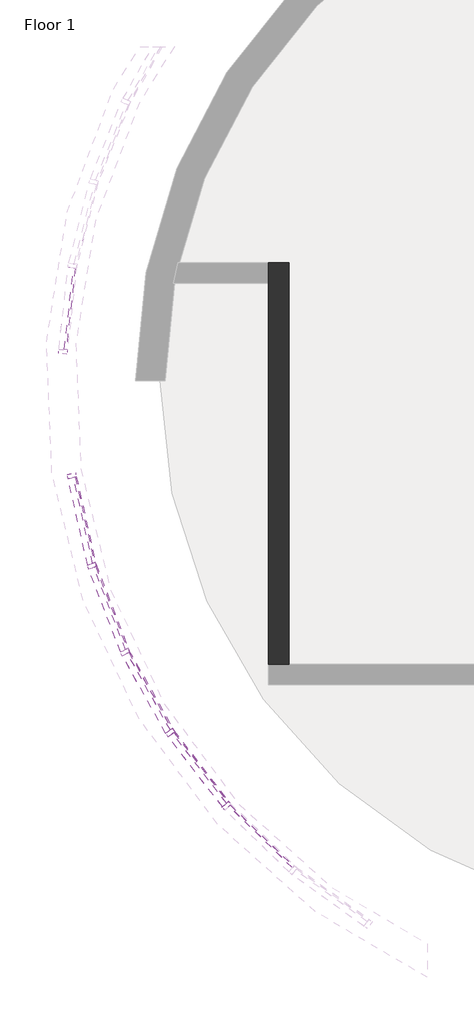
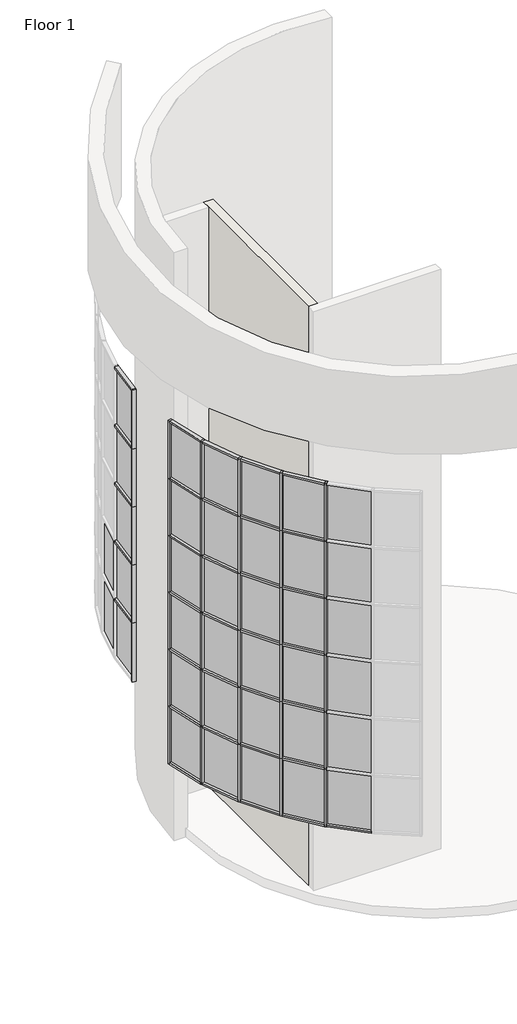
# One storey, part 1 of 11: 69 members, 37 plates, 1 wall.
"""IFC4 building model written with IfcOpenShell, lengths in millimetres."""

import ifcopenshell
import ifcopenshell.guid

model = None  # the IFC model being written
_history = None  # IfcOwnerHistory: only IFC2X3 demands one
_inside = {}  # id of a spatial element -> (the spatial element, [elements in it])
_under = {}  # id of a project, library or spatial element -> (it, [spatial elements below it])
_declared = {}  # id of a project -> (the project, [libraries it declares])
_typed = {}  # id of a type object -> (the type object, [elements of that type])
_made_of = {}  # id of a material, layer set ... -> (it, [elements and type objects made of it])


def new_model(schema):
    """Start an empty IFC model of exactly this schema.

    Asked for "IFC4X3", IfcOpenShell would pick the latest addendum, in which some entities
    have other attributes; the version numbers below select the first issue.
    IFC2X3 requires an IfcOwnerHistory on every rooted entity: one is made here for all.
    """
    global model, _history
    if schema == "IFC4X3":
        model = ifcopenshell.file(schema_version=(4, 3, 0, 0))
    else:
        model = ifcopenshell.file(schema=schema)
    _inside.clear()
    _under.clear()
    _declared.clear()
    _typed.clear()
    _made_of.clear()
    _history = None
    if model.schema == "IFC2X3":
        org = make("IfcOrganization", Name="unknown")
        user = make(
            "IfcPersonAndOrganization",
            ThePerson=make("IfcPerson", FamilyName="unknown"),
            TheOrganization=org,
        )
        app = make(
            "IfcApplication",
            ApplicationDeveloper=org,
            Version="unknown",
            ApplicationFullName="unknown",
            ApplicationIdentifier="unknown",
        )
        _history = make(
            "IfcOwnerHistory",
            OwningUser=user,
            OwningApplication=app,
            ChangeAction="ADDED",
            CreationDate=0,
        )
    return model


def make(cls, **values):
    """One entity of the class cls with the attributes given. An attribute that is None is left unset."""
    return model.create_entity(
        cls, **{name: value for name, value in values.items() if value is not None}
    )


def rooted(cls, **values):
    """An entity with a GlobalId (a new one), such as an element, a storey or a relation."""
    return make(cls, GlobalId=ifcopenshell.guid.new(), OwnerHistory=_history, **values)


def si_unit(unit_type, name, prefix=None):
    """IfcSIUnit, for example si_unit("LENGTHUNIT", "METRE", prefix="MILLI")."""
    return make("IfcSIUnit", UnitType=unit_type, Prefix=prefix, Name=name)


def assignment(units):
    """IfcUnitAssignment: the units of a project."""
    return None if units is None else make("IfcUnitAssignment", Units=units)


def point(xyz):
    """IfcCartesianPoint."""
    return None if xyz is None else make("IfcCartesianPoint", Coordinates=xyz)


def direction(xyz):
    """IfcDirection."""
    return None if xyz is None else make("IfcDirection", DirectionRatios=xyz)


def frame(location, z_axis=None, x_axis=None):
    """IfcAxis2Placement3D, a coordinate frame: its origin and axes. An axis left out is left unset."""
    return make(
        "IfcAxis2Placement3D",
        Location=point(location),
        Axis=direction(z_axis),
        RefDirection=direction(x_axis),
    )


def origin():
    """The frame at (0, 0, 0) with its axes left unset."""
    return frame((0.0, 0.0, 0.0))


def origin_with_axes():
    """The frame at (0, 0, 0) with the z axis (0, 0, 1) and the x axis (1, 0, 0) written out."""
    return frame((0.0, 0.0, 0.0), z_axis=(0.0, 0.0, 1.0), x_axis=(1.0, 0.0, 0.0))


def place(relative_to, where):
    """IfcLocalPlacement: puts the frame where relative to a parent placement (None: the world)."""
    return make(
        "IfcLocalPlacement", PlacementRelTo=relative_to, RelativePlacement=where
    )


def context(
    kind, dimensions, precision=None, world=None, true_north=None, identifier=None
):
    """IfcGeometricRepresentationContext, for example the 3D "Model" context."""
    return make(
        "IfcGeometricRepresentationContext",
        ContextIdentifier=identifier,
        ContextType=kind,
        CoordinateSpaceDimension=dimensions,
        Precision=precision,
        WorldCoordinateSystem=world,
        TrueNorth=true_north,
    )


def project(units=None, contexts=None):
    """IfcProject with its units and contexts."""
    return rooted(
        "IfcProject",
        Name="project",
        RepresentationContexts=contexts,
        UnitsInContext=assignment(units),
    )


def spatial(cls, under=None, at=None, **own):
    """A site, building, storey or space (cls), placed at a placement, below another one or the project."""
    s = rooted(cls, ObjectPlacement=at, **own)
    if under is not None:
        _under.setdefault(under.id(), (under, []))[1].append(s)
    return s


def polyline(points):
    """IfcPolyline through the points."""
    return make("IfcPolyline", Points=[point(p) for p in points])


def outline(outer, holes=None, kind="AREA"):
    """IfcArbitraryClosedProfileDef: a profile drawn as a closed curve; with holes, ...WithVoids."""
    if holes is None:
        return make("IfcArbitraryClosedProfileDef", ProfileType=kind, OuterCurve=outer)
    return make(
        "IfcArbitraryProfileDefWithVoids",
        ProfileType=kind,
        OuterCurve=outer,
        InnerCurves=holes,
    )


def extrude(swept, where, along, depth):
    """IfcExtrudedAreaSolid: the profile swept, set in the frame where, extruded along a direction by depth."""
    return make(
        "IfcExtrudedAreaSolid",
        SweptArea=swept,
        Position=where,
        ExtrudedDirection=direction(along),
        Depth=depth,
    )


def faces_of(points, faces, orient=None, outer=None):
    """IfcFace entities. A face is a list of loops; a loop is a list of indices into points, from 0.

    orient and outer hold one flag for each loop. By default every Orientation is true, the
    first loop of a face is its IfcFaceOuterBound and the others are IfcFaceBound.
    """
    made = []
    for i, loops in enumerate(faces):
        bounds = []
        for j, loop in enumerate(loops):
            is_outer = j == 0 if outer is None else outer[i][j]
            bounds.append(
                make(
                    "IfcFaceOuterBound" if is_outer else "IfcFaceBound",
                    Bound=make("IfcPolyLoop", Polygon=[points[k] for k in loop]),
                    Orientation=True if orient is None else orient[i][j],
                )
            )
        made.append(make("IfcFace", Bounds=bounds))
    return made


def faceted_brep(points, faces, orient=None, outer=None, voids=None):
    """IfcFacetedBrep: a solid bounded by flat faces; with voids (closed shells), ...WithVoids."""
    shared = [point(p) for p in points]
    hull = make("IfcClosedShell", CfsFaces=faces_of(shared, faces, orient, outer))
    if voids is None:
        return make("IfcFacetedBrep", Outer=hull)
    return make(
        "IfcFacetedBrepWithVoids",
        Outer=hull,
        Voids=[
            make(cls, CfsFaces=faces_of(shared, fs, o, b)) for cls, fs, o, b in voids
        ],
    )


def shape(context_of_items, identifier, shape_type, items):
    """IfcShapeRepresentation: the items that make up one representation, for example the "Body"."""
    return make(
        "IfcShapeRepresentation",
        ContextOfItems=context_of_items,
        RepresentationIdentifier=identifier,
        RepresentationType=shape_type,
        Items=items,
    )


def source(mapping_origin, context_of_items, identifier, shape_type, items):
    """IfcRepresentationMap: a shape defined once, which mapped items show again and again."""
    return make(
        "IfcRepresentationMap",
        MappingOrigin=mapping_origin,
        MappedRepresentation=shape(context_of_items, identifier, shape_type, items),
    )


def transform(
    local_origin,
    x_axis=None,
    y_axis=None,
    z_axis=None,
    scale=None,
    scale2=None,
    scale3=None,
    uniform=True,
):
    """IfcCartesianTransformationOperator3D, or its non-uniform kind. x_axis, y_axis, z_axis: its Axis1, 2, 3."""
    if uniform:
        return make(
            "IfcCartesianTransformationOperator3D",
            Axis1=direction(x_axis),
            Axis2=direction(y_axis),
            LocalOrigin=point(local_origin),
            Scale=scale,
            Axis3=direction(z_axis),
        )
    return make(
        "IfcCartesianTransformationOperator3DnonUniform",
        Axis1=direction(x_axis),
        Axis2=direction(y_axis),
        LocalOrigin=point(local_origin),
        Scale=scale,
        Axis3=direction(z_axis),
        Scale2=scale2,
        Scale3=scale3,
    )


def mapped(mapping_source, mapping_target):
    """IfcMappedItem: shows the shape of a source again, moved by a transform."""
    return make(
        "IfcMappedItem", MappingSource=mapping_source, MappingTarget=mapping_target
    )


def made_of(thing, what):
    """Note that an element or type object is made of a material, layer set ...; save() writes the relation."""
    if what is not None:
        _made_of.setdefault(what.id(), (what, []))[1].append(thing)
    return thing


def element(
    cls,
    number,
    at=None,
    inside=None,
    cuts=None,
    type_object=None,
    material=None,
    context=None,
    identifier="Body",
    shape_type=None,
    held_by="IfcProductDefinitionShape",
    body=None,
    shapes=None,
    **own,
):
    """One element of the class cls, such as IfcWall. Its Tag is "e" and its number.

    at: its placement. inside: the storey or other place that contains it. cuts: it is an
    opening in that element (IfcRelVoidsElement). A single representation is given by context,
    identifier, shape_type and body (its items); several are given by shapes. held_by: the class
    of the entity that holds the representations. save() writes the other relations.
    """
    e = rooted(cls, Tag="e%d" % number, ObjectPlacement=at, **own)
    if body is not None:
        shapes = [shape(context, identifier, shape_type, body)]
    if shapes is not None:
        e.Representation = make(held_by, Representations=shapes)
    if inside is not None:
        _inside.setdefault(inside.id(), (inside, []))[1].append(e)
    if cuts is not None:
        rooted(
            "IfcRelVoidsElement", RelatingBuildingElement=cuts, RelatedOpeningElement=e
        )
    if type_object is not None:
        _typed.setdefault(type_object.id(), (type_object, []))[1].append(e)
    return made_of(e, material)


def aggregate(whole, parts):
    """IfcRelAggregates: a whole, such as a stair, and the parts it consists of."""
    return rooted("IfcRelAggregates", RelatingObject=whole, RelatedObjects=parts)


def save(model, path):
    """Write the relations noted so far, then the file.

    IfcRelAggregates (storeys below a building ...), IfcRelContainedInSpatialStructure (elements
    in a storey), IfcRelDefinesByType, IfcRelAssociatesMaterial and IfcRelDeclares: one each for
    every whole, place, type object, material and project.
    """
    for whole, parts in _under.values():
        aggregate(whole, parts)
    for where, things in _inside.values():
        rooted(
            "IfcRelContainedInSpatialStructure",
            RelatedElements=things,
            RelatingStructure=where,
        )
    for kind, things in _typed.values():
        rooted("IfcRelDefinesByType", RelatedObjects=things, RelatingType=kind)
    for what, things in _made_of.values():
        rooted("IfcRelAssociatesMaterial", RelatedObjects=things, RelatingMaterial=what)
    for by, libraries in _declared.values():
        rooted("IfcRelDeclares", RelatingContext=by, RelatedDefinitions=libraries)
    model.write(path)


def member_2ae322fc(model_context):
    return source(origin(), model_context, "Body", "SweptSolid", [
        extrude(outline(polyline([(-63.5, 0.0), (63.5, 0.0), (63.5, -1253.5867756), (-61.1522336, -1244.9455147), (-63.5, -1278.8126009), (-63.5, 0.0)])), frame((-63.5, 0.0, 0.0), z_axis=(1.0, 0.0, 0.0), x_axis=(0.0, 1.0, 0.0)), (0.0, 0.0, 1.0), 63.5),
    ])


def member_21287d99(model_context):
    return source(origin(), model_context, "Body", "Brep", [
        faceted_brep([(31.75, 63.5, 0.0), (-31.75, 63.5, 0.0), (-31.75, -63.5, 0.0), (31.75, -63.5, 0.0), (31.75, 63.5, -1253.5867756), (0.0, 63.5, -1253.5867756), (-31.75, 63.5, -1253.5867756), (-31.75, -61.1522336, -1244.9455147), (-31.75, -63.5, -1278.8126009), (0.0, -63.5, -1278.8126009), (31.75, -63.5, -1278.8126009), (31.75, -61.1522336, -1244.9455147), (0.0, -61.1522336, -1244.9455147)], [[[0, 1, 2, 3]], [[1, 0, 4, 5, 6]], [[2, 1, 6, 7, 8]], [[3, 2, 8, 9, 10]], [[0, 3, 10, 11, 4]], [[4, 11, 12, 5]], [[11, 10, 9, 12]], [[9, 8, 7, 12]], [[7, 6, 5, 12]]]),
    ])


def member_2f5ef470(model_context):
    return source(origin(), model_context, "Body", "SweptSolid", [
        extrude(outline(polyline([(-63.5, 0.0), (63.5, 0.0), (63.5, -1344.0500431), (-60.9736199, -1334.8041085), (-63.5, -1368.815562), (-63.5, 0.0)])), frame((-63.5, 0.0, 0.0), z_axis=(1.0, 0.0, 0.0), x_axis=(0.0, 1.0, 0.0)), (0.0, 0.0, 1.0), 63.5),
    ])


def member_58fb4e6d(model_context):
    return source(origin(), model_context, "Body", "SweptSolid", [
        extrude(outline(polyline([(-63.5, 29.3948455), (-60.9736199, -4.616608), (63.5, 4.6293267), (63.5, -1339.4207165), (-63.5, -1339.4207165), (-63.5, 29.3948455)])), frame((-63.5, 0.0, 0.0), z_axis=(1.0, 0.0, 0.0), x_axis=(0.0, 1.0, 0.0)), (0.0, 0.0, 1.0), 63.5),
    ])


def member_233ab79f(model_context):
    return source(origin(), model_context, "Body", "SweptSolid", [
        extrude(outline(polyline([(-63.5, 29.4471051), (-61.0333155, -4.5163328), (63.5, 4.5282284), (63.5, -1343.9489353), (-61.0333155, -1334.904374), (-63.5, -1368.8678119), (-63.5, 29.4471051)])), frame((-63.5, 0.0, 0.0), z_axis=(1.0, 0.0, 0.0), x_axis=(0.0, 1.0, 0.0)), (0.0, 0.0, 1.0), 63.5),
    ])


def member_23db0025(model_context):
    return source(origin(), model_context, "Body", "Brep", [
        faceted_brep([(31.75, 63.5, -1339.4207165), (31.75, -63.5, -1339.4207165), (-31.75, -63.5, -1339.4207165), (-31.75, 63.5, -1339.4207165), (-31.75, 63.5, 4.6293267), (0.0, 63.5, 4.6293267), (31.75, 63.5, 4.6293267), (-31.75, -63.5, 29.3948455), (-31.75, -60.9736199, -4.616608), (31.75, -63.5, 29.3948455), (0.0, -63.5, 29.3948455), (31.75, -60.9736199, -4.616608), (0.0, -60.9736199, -4.616608)], [[[0, 1, 2, 3]], [[4, 5, 6, 0, 3]], [[7, 8, 4, 3, 2]], [[9, 10, 7, 2, 1]], [[6, 11, 9, 1, 0]], [[6, 5, 12, 11]], [[5, 4, 8, 12]], [[8, 7, 10, 12]], [[10, 9, 11, 12]]]),
    ])


def member_995572cb(model_context):
    return source(origin(), model_context, "Body", "Brep", [
        faceted_brep([(-31.75, 63.5, 4.5282284), (0.0, 63.5, 4.5282284), (31.75, 63.5, 4.5282284), (31.75, 63.5, -1343.9489353), (0.0, 63.5, -1343.9489353), (-31.75, 63.5, -1343.9489353), (-31.75, -63.5, 29.4471051), (-31.75, -61.0333155, -4.5163328), (-31.75, -61.0333155, -1334.904374), (-31.75, -63.5, -1368.8678119), (31.75, -63.5, 29.4471051), (0.0, -63.5, 29.4471051), (0.0, -63.5, -1368.8678119), (31.75, -63.5, -1368.8678119), (31.75, -61.0333155, -4.5163328), (31.75, -61.0333155, -1334.904374), (0.0, -61.0333155, -4.5163328), (0.0, -61.0333155, -1334.904374)], [[[0, 1, 2, 3, 4, 5]], [[6, 7, 0, 5, 8, 9]], [[10, 11, 6, 9, 12, 13]], [[2, 14, 10, 13, 15, 3]], [[2, 1, 16, 14]], [[1, 0, 7, 16]], [[7, 6, 11, 16]], [[11, 10, 14, 16]], [[3, 15, 17, 4]], [[15, 13, 12, 17]], [[12, 9, 8, 17]], [[8, 5, 4, 17]]]),
    ])


def member_0efe1817(model_context):
    return source(origin(), model_context, "Body", "SweptSolid", [
        extrude(outline(polyline([(31.75, 63.5), (31.75, -63.5), (-31.75, -63.5), (-31.75, 63.5), (31.75, 63.5)])), frame((0.0, 0.0, -2053.1666667), z_axis=(0.0, 0.0, 1.0), x_axis=(1.0, 0.0, 0.0)), (0.0, 0.0, 1.0), 2053.1666667),
    ])


def member_5e46efc9(model_context):
    return source(origin(), model_context, "Body", "SweptSolid", [
        extrude(outline(polyline([(31.75, 63.5), (31.75, -63.5), (-31.75, -63.5), (-31.75, 63.5), (31.75, 63.5)])), frame((0.0, 0.0, -2021.4166667), z_axis=(0.0, 0.0, 1.0), x_axis=(1.0, 0.0, 0.0)), (0.0, 0.0, 1.0), 2021.4166667),
    ])


def member_a397286f(model_context):
    return source(origin(), model_context, "Body", "SweptSolid", [
        extrude(outline(polyline([(0.0, 63.5), (0.0, -63.5), (-63.5, -63.5), (-63.5, 63.5), (0.0, 63.5)])), frame((0.0, 0.0, -2091.69), z_axis=(0.0, 0.0, 1.0), x_axis=(1.0, 0.0, 0.0)), (0.0, 0.0, 1.0), 2091.69),
    ])


def member_60f5540e(model_context):
    return source(origin(), model_context, "Body", "SweptSolid", [
        extrude(outline(polyline([(0.0, 63.5), (0.0, -63.5), (-63.5, -63.5), (-63.5, 63.5), (0.0, 63.5)])), frame((0.0, 0.0, -2053.1666667), z_axis=(0.0, 0.0, 1.0), x_axis=(1.0, 0.0, 0.0)), (0.0, 0.0, 1.0), 2053.1666667),
    ])


def member_08becc7e(model_context):
    return source(origin(), model_context, "Body", "SweptSolid", [
        extrude(outline(polyline([(0.0, 63.5), (0.0, -63.5), (-63.5, -63.5), (-63.5, 63.5), (0.0, 63.5)])), frame((0.0, 0.0, -2059.94), z_axis=(0.0, 0.0, 1.0), x_axis=(1.0, 0.0, 0.0)), (0.0, 0.0, 1.0), 2059.94),
    ])


def member_3a2f4316(model_context):
    return source(origin(), model_context, "Body", "SweptSolid", [
        extrude(outline(polyline([(0.0, 63.5), (0.0, -63.5), (-63.5, -63.5), (-63.5, 63.5), (0.0, 63.5)])), frame((0.0, 0.0, -2021.4166667), z_axis=(0.0, 0.0, 1.0), x_axis=(1.0, 0.0, 0.0)), (0.0, 0.0, 1.0), 2021.4166667),
    ])


def system_panel_glazed_5cc509e3(model_context):
    return source(origin(), model_context, "Body", "SweptSolid", [
        extrude(outline(polyline([(624.6304833, 19.05), (-624.6304833, 19.05), (-624.6304833, 44.45), (624.6304833, 44.45), (624.6304833, 19.05)])), origin_with_axes(), (0.0, 0.0, 1.0), 1996.44),
    ])


def system_panel_glazed_c8739ac2(model_context):
    return source(origin(), model_context, "Body", "SweptSolid", [
        extrude(outline(polyline([(669.7103582, 19.05), (-669.7103582, 19.05), (-669.7103582, 44.45), (669.7103582, 44.45), (669.7103582, 19.05)])), origin_with_axes(), (0.0, 0.0, 1.0), 1957.9166667),
    ])


def system_panel_glazed_63f175b4(model_context):
    return source(origin(), model_context, "Body", "SweptSolid", [
        extrude(outline(polyline([(624.6304785, 19.05), (-624.6304785, 19.05), (-624.6304785, 44.45), (624.6304785, 44.45), (624.6304785, 19.05)])), origin_with_axes(), (0.0, 0.0, 1.0), 1996.44),
    ])


def system_panel_glazed_41482947(model_context):
    return source(origin(), model_context, "Body", "SweptSolid", [
        extrude(outline(polyline([(669.7103534, 19.05), (-669.7103534, 19.05), (-669.7103534, 44.45), (669.7103534, 44.45), (669.7103534, 19.05)])), origin_with_axes(), (0.0, 0.0, 1.0), 1957.9166667),
    ])


model = new_model("IFC4")

# Units and contexts
model_context = context("Model", 3, world=origin())
ifc_project = project(units=[si_unit("LENGTHUNIT", "METRE", prefix="MILLI")], contexts=[model_context])

# Site, building, storey
site = spatial("IfcSite", under=ifc_project)
building = spatial("IfcBuilding", under=site)
storey = spatial("IfcBuildingStorey", under=building, Name="Floor 1", Elevation=0.0)

# Members
placement = place(None, origin())
member_shape = member_2ae322fc(model_context)
element("IfcMember", 1, ObjectType="Rectangular Mullion1 : 2.5\" x 5\" rectangular", at=placement, inside=storey, context=model_context, shape_type="MappedRepresentation", body=[
    mapped(member_shape, transform((-3372.5370712, 19812.4001373, 15849.6), x_axis=(0.0, 0.0, 1.0), y_axis=(-0.9938242310683915, 0.11096575030756306, 0.0), z_axis=(-0.11096575030756306, -0.9938242310683915, 0.0))),
])
member_2_shape = member_21287d99(model_context)
element("IfcMember", 2, ObjectType="Rectangular Mullion1 : 2.5\" x 5\" rectangular", at=placement, inside=storey, context=model_context, shape_type="MappedRepresentation", body=[
    mapped(member_2_shape, transform((-3372.5370712, 19812.4001373, 7578.09), x_axis=(0.0, 0.0, 1.0), y_axis=(-0.9938242310683916, 0.11096575030756314, 0.0), z_axis=(-0.11096575030756314, -0.9938242310683916, 0.0))),
])
element("IfcMember", 3, ObjectType="Rectangular Mullion1 : 2.5\" x 5\" rectangular", at=placement, inside=storey, context=model_context, shape_type="MappedRepresentation", body=[
    mapped(member_2_shape, transform((-3372.5370712, 19812.4001373, 9638.03), x_axis=(0.0, 0.0, 1.0), y_axis=(-0.9938242310683916, 0.11096575030756314, 0.0), z_axis=(-0.11096575030756314, -0.9938242310683916, 0.0))),
])
element("IfcMember", 4, ObjectType="Rectangular Mullion1 : 2.5\" x 5\" rectangular", at=placement, inside=storey, context=model_context, shape_type="MappedRepresentation", body=[
    mapped(member_2_shape, transform((-3372.5370712, 19812.4001373, 11697.97), x_axis=(0.0, 0.0, 1.0), y_axis=(-0.9938242310683916, 0.11096575030756314, 0.0), z_axis=(-0.11096575030756314, -0.9938242310683916, 0.0))),
])
element("IfcMember", 5, ObjectType="Rectangular Mullion1 : 2.5\" x 5\" rectangular", at=placement, inside=storey, context=model_context, shape_type="MappedRepresentation", body=[
    mapped(member_2_shape, transform((-3372.5370712, 19812.4001373, 13757.91), x_axis=(0.0, 0.0, 1.0), y_axis=(-0.9938242310683916, 0.11096575030756314, 0.0), z_axis=(-0.11096575030756314, -0.9938242310683916, 0.0))),
])
member_3_shape = member_2f5ef470(model_context)
element("IfcMember", 6, ObjectType="Rectangular Mullion1 : 2.5\" x 5\" rectangular", at=placement, inside=storey, context=model_context, shape_type="MappedRepresentation", body=[
    mapped(member_3_shape, transform((-3234.0499823, 17868.9864839, 3657.6), x_axis=(0.0, 0.0, -1.0), y_axis=(-0.9758306446122771, -0.2185281515859865, 0.0), z_axis=(-0.21852815158598649, 0.975830644612277, 0.0))),
])
member_4_shape = member_58fb4e6d(model_context)
element("IfcMember", 7, ObjectType="Rectangular Mullion1 : 2.5\" x 5\" rectangular", at=placement, inside=storey, context=model_context, shape_type="MappedRepresentation", body=[
    mapped(member_4_shape, transform((-2941.3488489, 16561.9387028, 15849.6), x_axis=(0.0, 0.0, 1.0), y_axis=(-0.9758306446122771, -0.2185281515859865, 0.0), z_axis=(0.21852815158598649, -0.975830644612277, 0.0))),
])
member_5_shape = member_233ab79f(model_context)
element("IfcMember", 8, ObjectType="Rectangular Mullion1 : 2.5\" x 5\" rectangular", at=placement, inside=storey, context=model_context, shape_type="MappedRepresentation", body=[
    mapped(member_5_shape, transform((-2442.4749788, 15251.0699632, 15849.6), x_axis=(0.0, 0.0, 1.0), y_axis=(-0.9334258019208646, -0.3587705008893443, 0.0), z_axis=(0.35877050088934426, -0.9334258019208644, 0.0))),
])
element("IfcMember", 9, ObjectType="Rectangular Mullion1 : 2.5\" x 5\" rectangular", at=placement, inside=storey, context=model_context, shape_type="MappedRepresentation", body=[
    mapped(member_5_shape, transform((-1759.3761459, 14026.0602606, 15849.6), x_axis=(0.0, 0.0, 1.0), y_axis=(-0.8717903813664917, -0.4898790983057628, 0.0), z_axis=(0.48987909830576276, -0.8717903813664916, 0.0))),
])
element("IfcMember", 10, ObjectType="Rectangular Mullion1 : 2.5\" x 5\" rectangular", at=placement, inside=storey, context=model_context, shape_type="MappedRepresentation", body=[
    mapped(member_5_shape, transform((-906.4404132, 12912.6091289, 15849.6), x_axis=(0.0, 0.0, 1.0), y_axis=(-0.7918574848272819, -0.6107059224561452, 0.0), z_axis=(0.6107059224561452, -0.7918574848272819, 0.0))),
])
element("IfcMember", 11, ObjectType="Rectangular Mullion1 : 2.5\" x 5\" rectangular", at=placement, inside=storey, context=model_context, shape_type="MappedRepresentation", body=[
    mapped(member_5_shape, transform((-2923.0196167, 16501.3198106, 3657.6), x_axis=(0.0, 0.0, -1.0), y_axis=(-0.9334258019208646, -0.3587705008893443, 0.0), z_axis=(-0.3587705008893443, 0.9334258019208646, 0.0))),
])
element("IfcMember", 12, ObjectType="Rectangular Mullion1 : 2.5\" x 5\" rectangular", at=placement, inside=storey, context=model_context, shape_type="MappedRepresentation", body=[
    mapped(member_5_shape, transform((-2415.530354, 15193.7543494, 3657.6), x_axis=(0.0, 0.0, -1.0), y_axis=(-0.8717903813664916, -0.4898790983057628, 0.0), z_axis=(-0.4898790983057628, 0.8717903813664916, 0.0))),
])
element("IfcMember", 13, ObjectType="Rectangular Mullion1 : 2.5\" x 5\" rectangular", at=placement, inside=storey, context=model_context, shape_type="MappedRepresentation", body=[
    mapped(member_5_shape, transform((-1724.4325715, 13973.2394409, 3657.6), x_axis=(0.0, 0.0, -1.0), y_axis=(-0.7918574848272819, -0.6107059224561452, 0.0), z_axis=(-0.6107059224561452, 0.7918574848272819, 0.0))),
])
element("IfcMember", 14, ObjectType="Rectangular Mullion1 : 2.5\" x 5\" rectangular", at=placement, inside=storey, context=model_context, shape_type="MappedRepresentation", body=[
    mapped(member_5_shape, transform((-864.2312985, 12865.3917271, 3657.6), x_axis=(0.0, 0.0, -1.0), y_axis=(-0.6953047750603438, -0.7187150129072613, 0.0), z_axis=(-0.7187150129072613, 0.6953047750603438, 0.0))),
])
member_6_shape = member_23db0025(model_context)
element("IfcMember", 15, ObjectType="Rectangular Mullion1 : 2.5\" x 5\" rectangular", at=placement, inside=storey, context=model_context, shape_type="MappedRepresentation", body=[
    mapped(member_6_shape, transform((-2941.3488489, 16561.9387028, 5710.7666667), x_axis=(0.0, 0.0, 1.0), y_axis=(-0.9758306446122771, -0.2185281515859863, 0.0), z_axis=(0.2185281515859863, -0.9758306446122771, 0.0))),
])
member_7_shape = member_995572cb(model_context)
element("IfcMember", 16, ObjectType="Rectangular Mullion1 : 2.5\" x 5\" rectangular", at=placement, inside=storey, context=model_context, shape_type="MappedRepresentation", body=[
    mapped(member_7_shape, transform((-2442.4749788, 15251.0699632, 5710.7666667), x_axis=(0.0, 0.0, 1.0), y_axis=(-0.9334258019208646, -0.3587705008893443, 0.0), z_axis=(0.35877050088934426, -0.9334258019208644, 0.0))),
])
element("IfcMember", 17, ObjectType="Rectangular Mullion1 : 2.5\" x 5\" rectangular", at=placement, inside=storey, context=model_context, shape_type="MappedRepresentation", body=[
    mapped(member_7_shape, transform((-1759.3761459, 14026.0602606, 5710.7666667), x_axis=(0.0, 0.0, 1.0), y_axis=(-0.8717903813664916, -0.4898790983057628, 0.0), z_axis=(0.4898790983057628, -0.8717903813664916, 0.0))),
])
element("IfcMember", 18, ObjectType="Rectangular Mullion1 : 2.5\" x 5\" rectangular", at=placement, inside=storey, context=model_context, shape_type="MappedRepresentation", body=[
    mapped(member_7_shape, transform((-906.4404132, 12912.6091289, 5710.7666667), x_axis=(0.0, 0.0, 1.0), y_axis=(-0.7918574848272818, -0.6107059224561452, 0.0), z_axis=(0.6107059224561452, -0.7918574848272818, 0.0))),
])
element("IfcMember", 19, ObjectType="Rectangular Mullion1 : 2.5\" x 5\" rectangular", at=placement, inside=storey, context=model_context, shape_type="MappedRepresentation", body=[
    mapped(member_6_shape, transform((-2941.3488489, 16561.9387028, 7732.1833333), x_axis=(0.0, 0.0, 1.0), y_axis=(-0.9758306446122771, -0.2185281515859863, 0.0), z_axis=(0.2185281515859863, -0.9758306446122771, 0.0))),
])
element("IfcMember", 20, ObjectType="Rectangular Mullion1 : 2.5\" x 5\" rectangular", at=placement, inside=storey, context=model_context, shape_type="MappedRepresentation", body=[
    mapped(member_6_shape, transform((-2941.3488489, 16561.9387028, 9753.6), x_axis=(0.0, 0.0, 1.0), y_axis=(-0.9758306446122771, -0.2185281515859863, 0.0), z_axis=(0.2185281515859863, -0.9758306446122771, 0.0))),
])
element("IfcMember", 21, ObjectType="Rectangular Mullion1 : 2.5\" x 5\" rectangular", at=placement, inside=storey, context=model_context, shape_type="MappedRepresentation", body=[
    mapped(member_6_shape, transform((-2941.3488489, 16561.9387028, 11775.0166667), x_axis=(0.0, 0.0, 1.0), y_axis=(-0.9758306446122771, -0.2185281515859863, 0.0), z_axis=(0.2185281515859863, -0.9758306446122771, 0.0))),
])
element("IfcMember", 22, ObjectType="Rectangular Mullion1 : 2.5\" x 5\" rectangular", at=placement, inside=storey, context=model_context, shape_type="MappedRepresentation", body=[
    mapped(member_7_shape, transform((-2442.4749788, 15251.0699632, 7732.1833333), x_axis=(0.0, 0.0, 1.0), y_axis=(-0.9334258019208646, -0.3587705008893443, 0.0), z_axis=(0.35877050088934426, -0.9334258019208644, 0.0))),
])
element("IfcMember", 23, ObjectType="Rectangular Mullion1 : 2.5\" x 5\" rectangular", at=placement, inside=storey, context=model_context, shape_type="MappedRepresentation", body=[
    mapped(member_7_shape, transform((-1759.3761459, 14026.0602606, 7732.1833333), x_axis=(0.0, 0.0, 1.0), y_axis=(-0.8717903813664916, -0.489879098305763, 0.0), z_axis=(0.489879098305763, -0.8717903813664916, 0.0))),
])
element("IfcMember", 24, ObjectType="Rectangular Mullion1 : 2.5\" x 5\" rectangular", at=placement, inside=storey, context=model_context, shape_type="MappedRepresentation", body=[
    mapped(member_7_shape, transform((-906.4404132, 12912.6091289, 7732.1833333), x_axis=(0.0, 0.0, 1.0), y_axis=(-0.7918574848272818, -0.6107059224561452, 0.0), z_axis=(0.6107059224561452, -0.7918574848272818, 0.0))),
])
element("IfcMember", 25, ObjectType="Rectangular Mullion1 : 2.5\" x 5\" rectangular", at=placement, inside=storey, context=model_context, shape_type="MappedRepresentation", body=[
    mapped(member_7_shape, transform((-2442.4749788, 15251.0699632, 9753.6), x_axis=(0.0, 0.0, 1.0), y_axis=(-0.9334258019208646, -0.3587705008893443, 0.0), z_axis=(0.35877050088934426, -0.9334258019208644, 0.0))),
])
element("IfcMember", 26, ObjectType="Rectangular Mullion1 : 2.5\" x 5\" rectangular", at=placement, inside=storey, context=model_context, shape_type="MappedRepresentation", body=[
    mapped(member_7_shape, transform((-1759.3761459, 14026.0602606, 9753.6), x_axis=(0.0, 0.0, 1.0), y_axis=(-0.8717903813664917, -0.4898790983057627, 0.0), z_axis=(0.48987909830576265, -0.8717903813664916, 0.0))),
])
element("IfcMember", 27, ObjectType="Rectangular Mullion1 : 2.5\" x 5\" rectangular", at=placement, inside=storey, context=model_context, shape_type="MappedRepresentation", body=[
    mapped(member_7_shape, transform((-906.4404132, 12912.6091289, 9753.6), x_axis=(0.0, 0.0, 1.0), y_axis=(-0.7918574848272818, -0.6107059224561452, 0.0), z_axis=(0.6107059224561452, -0.7918574848272818, 0.0))),
])
element("IfcMember", 28, ObjectType="Rectangular Mullion1 : 2.5\" x 5\" rectangular", at=placement, inside=storey, context=model_context, shape_type="MappedRepresentation", body=[
    mapped(member_7_shape, transform((-2442.4749788, 15251.0699632, 11775.0166667), x_axis=(0.0, 0.0, 1.0), y_axis=(-0.9334258019208646, -0.3587705008893443, 0.0), z_axis=(0.35877050088934426, -0.9334258019208644, 0.0))),
])
element("IfcMember", 29, ObjectType="Rectangular Mullion1 : 2.5\" x 5\" rectangular", at=placement, inside=storey, context=model_context, shape_type="MappedRepresentation", body=[
    mapped(member_7_shape, transform((-1759.3761459, 14026.0602606, 11775.0166667), x_axis=(0.0, 0.0, 1.0), y_axis=(-0.8717903813664917, -0.4898790983057627, 0.0), z_axis=(0.48987909830576265, -0.8717903813664916, 0.0))),
])
element("IfcMember", 30, ObjectType="Rectangular Mullion1 : 2.5\" x 5\" rectangular", at=placement, inside=storey, context=model_context, shape_type="MappedRepresentation", body=[
    mapped(member_7_shape, transform((-906.4404132, 12912.6091289, 11775.0166667), x_axis=(0.0, 0.0, 1.0), y_axis=(-0.7918574848272818, -0.6107059224561452, 0.0), z_axis=(0.6107059224561452, -0.7918574848272818, 0.0))),
])
element("IfcMember", 31, ObjectType="Rectangular Mullion1 : 2.5\" x 5\" rectangular", at=placement, inside=storey, context=model_context, shape_type="MappedRepresentation", body=[
    mapped(member_6_shape, transform((-2941.3488489, 16561.9387028, 13796.4333333), x_axis=(0.0, 0.0, 1.0), y_axis=(-0.9758306446122771, -0.2185281515859865, 0.0), z_axis=(0.21852815158598649, -0.975830644612277, 0.0))),
])
element("IfcMember", 32, ObjectType="Rectangular Mullion1 : 2.5\" x 5\" rectangular", at=placement, inside=storey, context=model_context, shape_type="MappedRepresentation", body=[
    mapped(member_7_shape, transform((-2442.4749788, 15251.0699632, 13796.4333333), x_axis=(0.0, 0.0, 1.0), y_axis=(-0.9334258019208646, -0.3587705008893443, 0.0), z_axis=(0.35877050088934426, -0.9334258019208644, 0.0))),
])
element("IfcMember", 33, ObjectType="Rectangular Mullion1 : 2.5\" x 5\" rectangular", at=placement, inside=storey, context=model_context, shape_type="MappedRepresentation", body=[
    mapped(member_7_shape, transform((-1759.3761459, 14026.0602606, 13796.4333333), x_axis=(0.0, 0.0, 1.0), y_axis=(-0.8717903813664917, -0.4898790983057627, 0.0), z_axis=(0.48987909830576265, -0.8717903813664916, 0.0))),
])
element("IfcMember", 34, ObjectType="Rectangular Mullion1 : 2.5\" x 5\" rectangular", at=placement, inside=storey, context=model_context, shape_type="MappedRepresentation", body=[
    mapped(member_7_shape, transform((-906.4404132, 12912.6091289, 13796.4333333), x_axis=(0.0, 0.0, 1.0), y_axis=(-0.7918574848272818, -0.6107059224561452, 0.0), z_axis=(0.6107059224561452, -0.7918574848272818, 0.0))),
])
member_8_shape = member_0efe1817(model_context)
element("IfcMember", 35, ObjectType="Rectangular Mullion1 : 2.5\" x 5\" rectangular", at=placement, inside=storey, context=model_context, shape_type="MappedRepresentation", body=[
    mapped(member_8_shape, transform((-2934.4105801, 16530.9560798, 3657.6), x_axis=(0.2902135855625472, -0.9569618982775282, 0.0), y_axis=(-0.9569618982775282, -0.2902135855625472, 0.0), z_axis=(0.0, 0.0, -1.0))),
])
element("IfcMember", 36, ObjectType="Rectangular Mullion1 : 2.5\" x 5\" rectangular", at=placement, inside=storey, context=model_context, shape_type="MappedRepresentation", body=[
    mapped(member_8_shape, transform((-2431.0840154, 15221.433694, 3657.6), x_axis=(0.42544243655309744, -0.9049854878282655, 0.0), y_axis=(-0.9049854878282655, -0.42544243655309744, 0.0), z_axis=(0.0, 0.0, -1.0))),
])
element("IfcMember", 37, ObjectType="Rectangular Mullion1 : 2.5\" x 5\" rectangular", at=placement, inside=storey, context=model_context, shape_type="MappedRepresentation", body=[
    mapped(member_8_shape, transform((-1743.8224845, 13998.380916, 3657.6), x_axis=(0.5517419360250448, -0.8340148895741223, 0.0), y_axis=(-0.8340148895741223, -0.5517419360250448, 0.0), z_axis=(0.0, 0.0, -1.0))),
])
element("IfcMember", 38, ObjectType="Rectangular Mullion1 : 2.5\" x 5\" rectangular", at=placement, inside=storey, context=model_context, shape_type="MappedRepresentation", body=[
    mapped(member_8_shape, transform((-887.0505002, 12887.4676537, 3657.6), x_axis=(0.6664612609045398, -0.7455396620660306, 0.0), y_axis=(-0.7455396620660306, -0.6664612609045398, 0.0), z_axis=(0.0, 0.0, -1.0))),
])
member_9_shape = member_5e46efc9(model_context)
element("IfcMember", 39, ObjectType="Rectangular Mullion1 : 2.5\" x 5\" rectangular", at=placement, inside=storey, context=model_context, shape_type="MappedRepresentation", body=[
    mapped(member_9_shape, transform((-2934.4105801, 16530.9560798, 5710.7666667), x_axis=(0.2902135855625481, -0.9569618982775279, 0.0), y_axis=(-0.9569618982775279, -0.2902135855625481, 0.0), z_axis=(0.0, 0.0, -1.0))),
])
element("IfcMember", 40, ObjectType="Rectangular Mullion1 : 2.5\" x 5\" rectangular", at=placement, inside=storey, context=model_context, shape_type="MappedRepresentation", body=[
    mapped(member_9_shape, transform((-2431.0840154, 15221.433694, 5710.7666667), x_axis=(0.4254424365530983, -0.9049854878282652, 0.0), y_axis=(-0.9049854878282652, -0.4254424365530983, 0.0), z_axis=(0.0, 0.0, -1.0))),
])
element("IfcMember", 41, ObjectType="Rectangular Mullion1 : 2.5\" x 5\" rectangular", at=placement, inside=storey, context=model_context, shape_type="MappedRepresentation", body=[
    mapped(member_9_shape, transform((-1743.8224845, 13998.380916, 5710.7666667), x_axis=(0.5517419360250448, -0.8340148895741223, 0.0), y_axis=(-0.8340148895741223, -0.5517419360250448, 0.0), z_axis=(0.0, 0.0, -1.0))),
])
element("IfcMember", 42, ObjectType="Rectangular Mullion1 : 2.5\" x 5\" rectangular", at=placement, inside=storey, context=model_context, shape_type="MappedRepresentation", body=[
    mapped(member_9_shape, transform((-887.0505002, 12887.4676537, 5710.7666667), x_axis=(0.6664612609045398, -0.7455396620660306, 0.0), y_axis=(-0.7455396620660306, -0.6664612609045398, 0.0), z_axis=(0.0, 0.0, -1.0))),
])
element("IfcMember", 43, ObjectType="Rectangular Mullion1 : 2.5\" x 5\" rectangular", at=placement, inside=storey, context=model_context, shape_type="MappedRepresentation", body=[
    mapped(member_9_shape, transform((-2934.4105801, 16530.9560798, 7732.1833333), x_axis=(0.2902135855625481, -0.9569618982775279, 0.0), y_axis=(-0.9569618982775279, -0.2902135855625481, 0.0), z_axis=(0.0, 0.0, -1.0))),
])
element("IfcMember", 44, ObjectType="Rectangular Mullion1 : 2.5\" x 5\" rectangular", at=placement, inside=storey, context=model_context, shape_type="MappedRepresentation", body=[
    mapped(member_9_shape, transform((-2431.0840154, 15221.433694, 7732.1833333), x_axis=(0.4254424365530983, -0.9049854878282652, 0.0), y_axis=(-0.9049854878282652, -0.4254424365530983, 0.0), z_axis=(0.0, 0.0, -1.0))),
])
element("IfcMember", 45, ObjectType="Rectangular Mullion1 : 2.5\" x 5\" rectangular", at=placement, inside=storey, context=model_context, shape_type="MappedRepresentation", body=[
    mapped(member_9_shape, transform((-1743.8224845, 13998.380916, 7732.1833333), x_axis=(0.5517419360250448, -0.8340148895741223, 0.0), y_axis=(-0.8340148895741223, -0.5517419360250448, 0.0), z_axis=(0.0, 0.0, -1.0))),
])
element("IfcMember", 46, ObjectType="Rectangular Mullion1 : 2.5\" x 5\" rectangular", at=placement, inside=storey, context=model_context, shape_type="MappedRepresentation", body=[
    mapped(member_9_shape, transform((-887.0505002, 12887.4676537, 7732.1833333), x_axis=(0.6664612609045398, -0.7455396620660306, 0.0), y_axis=(-0.7455396620660306, -0.6664612609045398, 0.0), z_axis=(0.0, 0.0, -1.0))),
])
element("IfcMember", 47, ObjectType="Rectangular Mullion1 : 2.5\" x 5\" rectangular", at=placement, inside=storey, context=model_context, shape_type="MappedRepresentation", body=[
    mapped(member_9_shape, transform((-2934.4105801, 16530.9560798, 9753.6), x_axis=(0.2902135855625481, -0.9569618982775279, 0.0), y_axis=(-0.9569618982775279, -0.2902135855625481, 0.0), z_axis=(0.0, 0.0, -1.0))),
])
element("IfcMember", 48, ObjectType="Rectangular Mullion1 : 2.5\" x 5\" rectangular", at=placement, inside=storey, context=model_context, shape_type="MappedRepresentation", body=[
    mapped(member_9_shape, transform((-2431.0840154, 15221.433694, 9753.6), x_axis=(0.4254424365530983, -0.9049854878282652, 0.0), y_axis=(-0.9049854878282652, -0.4254424365530983, 0.0), z_axis=(0.0, 0.0, -1.0))),
])
element("IfcMember", 49, ObjectType="Rectangular Mullion1 : 2.5\" x 5\" rectangular", at=placement, inside=storey, context=model_context, shape_type="MappedRepresentation", body=[
    mapped(member_9_shape, transform((-1743.8224845, 13998.380916, 9753.6), x_axis=(0.5517419360250456, -0.8340148895741218, 0.0), y_axis=(-0.8340148895741218, -0.5517419360250456, 0.0), z_axis=(0.0, 0.0, -1.0))),
])
element("IfcMember", 50, ObjectType="Rectangular Mullion1 : 2.5\" x 5\" rectangular", at=placement, inside=storey, context=model_context, shape_type="MappedRepresentation", body=[
    mapped(member_9_shape, transform((-887.0505002, 12887.4676537, 9753.6), x_axis=(0.6664612609045398, -0.7455396620660306, 0.0), y_axis=(-0.7455396620660306, -0.6664612609045398, 0.0), z_axis=(0.0, 0.0, -1.0))),
])
element("IfcMember", 51, ObjectType="Rectangular Mullion1 : 2.5\" x 5\" rectangular", at=placement, inside=storey, context=model_context, shape_type="MappedRepresentation", body=[
    mapped(member_9_shape, transform((-2934.4105801, 16530.9560798, 11775.0166667), x_axis=(0.2902135855625481, -0.9569618982775279, 0.0), y_axis=(-0.9569618982775279, -0.2902135855625481, 0.0), z_axis=(0.0, 0.0, -1.0))),
])
element("IfcMember", 52, ObjectType="Rectangular Mullion1 : 2.5\" x 5\" rectangular", at=placement, inside=storey, context=model_context, shape_type="MappedRepresentation", body=[
    mapped(member_9_shape, transform((-2431.0840154, 15221.433694, 11775.0166667), x_axis=(0.4254424365530983, -0.9049854878282652, 0.0), y_axis=(-0.9049854878282652, -0.4254424365530983, 0.0), z_axis=(0.0, 0.0, -1.0))),
])
element("IfcMember", 53, ObjectType="Rectangular Mullion1 : 2.5\" x 5\" rectangular", at=placement, inside=storey, context=model_context, shape_type="MappedRepresentation", body=[
    mapped(member_9_shape, transform((-1743.8224845, 13998.380916, 11775.0166667), x_axis=(0.5517419360250456, -0.8340148895741218, 0.0), y_axis=(-0.8340148895741218, -0.5517419360250456, 0.0), z_axis=(0.0, 0.0, -1.0))),
])
element("IfcMember", 54, ObjectType="Rectangular Mullion1 : 2.5\" x 5\" rectangular", at=placement, inside=storey, context=model_context, shape_type="MappedRepresentation", body=[
    mapped(member_9_shape, transform((-887.0505002, 12887.4676537, 11775.0166667), x_axis=(0.6664612609045398, -0.7455396620660306, 0.0), y_axis=(-0.7455396620660306, -0.6664612609045398, 0.0), z_axis=(0.0, 0.0, -1.0))),
])
element("IfcMember", 55, ObjectType="Rectangular Mullion1 : 2.5\" x 5\" rectangular", at=placement, inside=storey, context=model_context, shape_type="MappedRepresentation", body=[
    mapped(member_8_shape, transform((-2934.4105801, 16530.9560798, 13796.4333333), x_axis=(0.2902135855625472, -0.9569618982775282, 0.0), y_axis=(-0.9569618982775282, -0.2902135855625472, 0.0), z_axis=(0.0, 0.0, -1.0))),
])
element("IfcMember", 56, ObjectType="Rectangular Mullion1 : 2.5\" x 5\" rectangular", at=placement, inside=storey, context=model_context, shape_type="MappedRepresentation", body=[
    mapped(member_8_shape, transform((-2431.0840154, 15221.433694, 13796.4333333), x_axis=(0.4254424365530983, -0.9049854878282652, 0.0), y_axis=(-0.9049854878282652, -0.4254424365530983, 0.0), z_axis=(0.0, 0.0, -1.0))),
])
element("IfcMember", 57, ObjectType="Rectangular Mullion1 : 2.5\" x 5\" rectangular", at=placement, inside=storey, context=model_context, shape_type="MappedRepresentation", body=[
    mapped(member_8_shape, transform((-1743.8224845, 13998.380916, 13796.4333333), x_axis=(0.5517419360250456, -0.8340148895741218, 0.0), y_axis=(-0.8340148895741218, -0.5517419360250456, 0.0), z_axis=(0.0, 0.0, -1.0))),
])
element("IfcMember", 58, ObjectType="Rectangular Mullion1 : 2.5\" x 5\" rectangular", at=placement, inside=storey, context=model_context, shape_type="MappedRepresentation", body=[
    mapped(member_8_shape, transform((-887.0505002, 12887.4676537, 13796.4333333), x_axis=(0.6664612609045398, -0.7455396620660306, 0.0), y_axis=(-0.7455396620660306, -0.6664612609045398, 0.0), z_axis=(0.0, 0.0, -1.0))),
])
member_10_shape = member_a397286f(model_context)
element("IfcMember", 59, ObjectType="Rectangular Mullion1 : 2.5\" x 5\" rectangular", at=placement, inside=storey, context=model_context, shape_type="MappedRepresentation", body=[
    mapped(member_10_shape, transform((-3379.5833964, 19749.2922986, 5486.4), x_axis=(-0.11096575030756324, -0.9938242310683915, 0.0), y_axis=(-0.9938242310683915, 0.11096575030756324, 0.0), z_axis=(0.0, 0.0, -1.0))),
])
member_11_shape = member_60f5540e(model_context)
element("IfcMember", 60, ObjectType="Rectangular Mullion1 : 2.5\" x 5\" rectangular", at=placement, inside=storey, context=model_context, shape_type="MappedRepresentation", body=[
    mapped(member_11_shape, transform((-3247.9265199, 17930.9517299, 15849.6), x_axis=(-0.21852815158598635, 0.9758306446122771, 0.0), y_axis=(-0.9758306446122771, -0.21852815158598635, 0.0), z_axis=(0.0, 0.0, 1.0))),
])
member_12_shape = member_08becc7e(model_context)
element("IfcMember", 61, ObjectType="Rectangular Mullion1 : 2.5\" x 5\" rectangular", at=placement, inside=storey, context=model_context, shape_type="MappedRepresentation", body=[
    mapped(member_12_shape, transform((-3379.5833964, 19749.2922986, 7578.09), x_axis=(-0.11096575030756325, -0.9938242310683915, 0.0), y_axis=(-0.9938242310683915, 0.11096575030756325, 0.0), z_axis=(0.0, 0.0, -1.0))),
])
element("IfcMember", 62, ObjectType="Rectangular Mullion1 : 2.5\" x 5\" rectangular", at=placement, inside=storey, context=model_context, shape_type="MappedRepresentation", body=[
    mapped(member_12_shape, transform((-3379.5833964, 19749.2922986, 9638.03), x_axis=(-0.11096575030756324, -0.9938242310683915, 0.0), y_axis=(-0.9938242310683915, 0.11096575030756324, 0.0), z_axis=(0.0, 0.0, -1.0))),
])
element("IfcMember", 63, ObjectType="Rectangular Mullion1 : 2.5\" x 5\" rectangular", at=placement, inside=storey, context=model_context, shape_type="MappedRepresentation", body=[
    mapped(member_12_shape, transform((-3379.5833964, 19749.2922986, 11697.97), x_axis=(-0.11096575030756324, -0.9938242310683915, 0.0), y_axis=(-0.9938242310683915, 0.11096575030756324, 0.0), z_axis=(0.0, 0.0, -1.0))),
])
element("IfcMember", 64, ObjectType="Rectangular Mullion1 : 2.5\" x 5\" rectangular", at=placement, inside=storey, context=model_context, shape_type="MappedRepresentation", body=[
    mapped(member_10_shape, transform((-3379.5833964, 19749.2922986, 13757.91), x_axis=(-0.11096575030756325, -0.9938242310683915, 0.0), y_axis=(-0.9938242310683915, 0.11096575030756325, 0.0), z_axis=(0.0, 0.0, -1.0))),
])
element("IfcMember", 65, ObjectType="Rectangular Mullion1 : 2.5\" x 5\" rectangular", at=placement, inside=storey, context=model_context, shape_type="MappedRepresentation", body=[
    mapped(member_11_shape, transform((-3247.9265199, 17930.9517299, 5710.7666667), x_axis=(-0.21852815158598632, 0.9758306446122771, 0.0), y_axis=(-0.9758306446122771, -0.21852815158598632, 0.0), z_axis=(0.0, 0.0, 1.0))),
])
member_13_shape = member_3a2f4316(model_context)
element("IfcMember", 66, ObjectType="Rectangular Mullion1 : 2.5\" x 5\" rectangular", at=placement, inside=storey, context=model_context, shape_type="MappedRepresentation", body=[
    mapped(member_13_shape, transform((-3247.9265199, 17930.9517299, 7732.1833333), x_axis=(-0.21852815158598632, 0.9758306446122771, 0.0), y_axis=(-0.9758306446122771, -0.21852815158598632, 0.0), z_axis=(0.0, 0.0, 1.0))),
])
element("IfcMember", 67, ObjectType="Rectangular Mullion1 : 2.5\" x 5\" rectangular", at=placement, inside=storey, context=model_context, shape_type="MappedRepresentation", body=[
    mapped(member_13_shape, transform((-3247.9265199, 17930.9517299, 9753.6), x_axis=(-0.21852815158598632, 0.9758306446122771, 0.0), y_axis=(-0.9758306446122771, -0.21852815158598632, 0.0), z_axis=(0.0, 0.0, 1.0))),
])
element("IfcMember", 68, ObjectType="Rectangular Mullion1 : 2.5\" x 5\" rectangular", at=placement, inside=storey, context=model_context, shape_type="MappedRepresentation", body=[
    mapped(member_13_shape, transform((-3247.9265199, 17930.9517299, 11775.0166667), x_axis=(-0.21852815158598632, 0.9758306446122771, 0.0), y_axis=(-0.9758306446122771, -0.21852815158598632, 0.0), z_axis=(0.0, 0.0, 1.0))),
])
element("IfcMember", 69, ObjectType="Rectangular Mullion1 : 2.5\" x 5\" rectangular", at=placement, inside=storey, context=model_context, shape_type="MappedRepresentation", body=[
    mapped(member_13_shape, transform((-3247.9265199, 17930.9517299, 13796.4333333), x_axis=(-0.21852815158598632, 0.9758306446122771, 0.0), y_axis=(-0.9758306446122771, -0.21852815158598632, 0.0), z_axis=(0.0, 0.0, 1.0))),
])

# Plates
system_panel_glazed_shape = system_panel_glazed_5cc509e3(model_context)
element("IfcPlate", 70, ObjectType="System Panel : Glazed", at=placement, inside=storey, context=model_context, shape_type="MappedRepresentation", body=[
    mapped(system_panel_glazed_shape, transform((-3303.224481, 20433.1730471, 5549.9), x_axis=(-0.11096575030756324, -0.9938242310683915, 0.0), y_axis=(0.9938242310683915, -0.11096575030756324, 0.0), z_axis=(0.0, 0.0, 1.0))),
])
element("IfcPlate", 71, ObjectType="System Panel : Glazed", at=placement, inside=storey, context=model_context, shape_type="MappedRepresentation", body=[
    mapped(system_panel_glazed_shape, transform((-3303.224481, 20433.1730471, 7609.84), x_axis=(-0.11096575030756325, -0.9938242310683915, 0.0), y_axis=(0.9938242310683915, -0.11096575030756325, 0.0), z_axis=(0.0, 0.0, 1.0))),
])
element("IfcPlate", 72, ObjectType="System Panel : Glazed", at=placement, inside=storey, context=model_context, shape_type="MappedRepresentation", body=[
    mapped(system_panel_glazed_shape, transform((-3303.224481, 20433.1730471, 9669.78), x_axis=(-0.11096575030756324, -0.9938242310683915, 0.0), y_axis=(0.9938242310683915, -0.11096575030756324, 0.0), z_axis=(0.0, 0.0, 1.0))),
])
element("IfcPlate", 73, ObjectType="System Panel : Glazed", at=placement, inside=storey, context=model_context, shape_type="MappedRepresentation", body=[
    mapped(system_panel_glazed_shape, transform((-3303.224481, 20433.1730471, 11729.72), x_axis=(-0.11096575030756324, -0.9938242310683915, 0.0), y_axis=(0.9938242310683915, -0.11096575030756324, 0.0), z_axis=(0.0, 0.0, 1.0))),
])
element("IfcPlate", 74, ObjectType="System Panel : Glazed", at=placement, inside=storey, context=model_context, shape_type="MappedRepresentation", body=[
    mapped(system_panel_glazed_shape, transform((-3303.224481, 20433.1730471, 13789.66), x_axis=(-0.11096575030756325, -0.9938242310683915, 0.0), y_axis=(0.9938242310683915, -0.11096575030756325, 0.0), z_axis=(0.0, 0.0, 1.0))),
])
system_panel_glazed_2_shape = system_panel_glazed_c8739ac2(model_context)
element("IfcPlate", 75, ObjectType="System Panel : Glazed", at=placement, inside=storey, context=model_context, shape_type="MappedRepresentation", body=[
    mapped(system_panel_glazed_2_shape, transform((-3087.6994156, 17215.4625934, 3721.1), x_axis=(0.21852815158598632, -0.9758306446122771, 0.0), y_axis=(0.9758306446122771, 0.21852815158598632, 0.0), z_axis=(0.0, 0.0, 1.0))),
])
element("IfcPlate", 76, ObjectType="System Panel : Glazed", at=placement, inside=storey, context=model_context, shape_type="MappedRepresentation", body=[
    mapped(system_panel_glazed_2_shape, transform((-3087.6994156, 17215.4625934, 5742.5166667), x_axis=(0.21852815158598632, -0.9758306446122771, 0.0), y_axis=(0.9758306446122771, 0.21852815158598632, 0.0), z_axis=(0.0, 0.0, 1.0))),
])
element("IfcPlate", 77, ObjectType="System Panel : Glazed", at=placement, inside=storey, context=model_context, shape_type="MappedRepresentation", body=[
    mapped(system_panel_glazed_2_shape, transform((-3087.6994156, 17215.4625934, 7763.9333333), x_axis=(0.21852815158598632, -0.9758306446122771, 0.0), y_axis=(0.9758306446122771, 0.21852815158598632, 0.0), z_axis=(0.0, 0.0, 1.0))),
])
element("IfcPlate", 78, ObjectType="System Panel : Glazed", at=placement, inside=storey, context=model_context, shape_type="MappedRepresentation", body=[
    mapped(system_panel_glazed_2_shape, transform((-3087.6994156, 17215.4625934, 9785.35), x_axis=(0.21852815158598632, -0.9758306446122771, 0.0), y_axis=(0.9758306446122771, 0.21852815158598632, 0.0), z_axis=(0.0, 0.0, 1.0))),
])
element("IfcPlate", 79, ObjectType="System Panel : Glazed", at=placement, inside=storey, context=model_context, shape_type="MappedRepresentation", body=[
    mapped(system_panel_glazed_2_shape, transform((-3087.6994156, 17215.4625934, 11806.7666667), x_axis=(0.21852815158598632, -0.9758306446122771, 0.0), y_axis=(0.9758306446122771, 0.21852815158598632, 0.0), z_axis=(0.0, 0.0, 1.0))),
])
element("IfcPlate", 80, ObjectType="System Panel : Glazed", at=placement, inside=storey, context=model_context, shape_type="MappedRepresentation", body=[
    mapped(system_panel_glazed_2_shape, transform((-3087.6994156, 17215.4625934, 13828.1833333), x_axis=(0.21852815158598635, -0.9758306446122771, 0.0), y_axis=(0.9758306446122771, 0.21852815158598635, 0.0), z_axis=(0.0, 0.0, 1.0))),
])
system_panel_glazed_3_shape = system_panel_glazed_63f175b4(model_context)
element("IfcPlate", 81, ObjectType="System Panel : Glazed", at=placement, inside=storey, context=model_context, shape_type="MappedRepresentation", body=[
    mapped(system_panel_glazed_3_shape, transform((-3069.2811615, 21721.8014435, 5549.9), x_axis=(-0.24544844333089522, -0.9694096459528554, 0.0), y_axis=(0.9694096459528554, -0.24544844333089522, 0.0), z_axis=(0.0, 0.0, 1.0))),
])
element("IfcPlate", 82, ObjectType="System Panel : Glazed", at=placement, inside=storey, context=model_context, shape_type="MappedRepresentation", body=[
    mapped(system_panel_glazed_3_shape, transform((-3069.2811615, 21721.8014435, 7609.84), x_axis=(-0.2454484433308952, -0.9694096459528554, 0.0), y_axis=(0.9694096459528554, -0.2454484433308952, 0.0), z_axis=(0.0, 0.0, 1.0))),
])
system_panel_glazed_4_shape = system_panel_glazed_41482947(model_context)
element("IfcPlate", 83, ObjectType="System Panel : Glazed", at=placement, inside=storey, context=model_context, shape_type="MappedRepresentation", body=[
    mapped(system_panel_glazed_4_shape, transform((-2682.7472977, 15876.1948869, 3721.1), x_axis=(0.35877050088934437, -0.9334258019208644, 0.0), y_axis=(0.9334258019208644, 0.35877050088934437, 0.0), z_axis=(0.0, 0.0, 1.0))),
])
element("IfcPlate", 84, ObjectType="System Panel : Glazed", at=placement, inside=storey, context=model_context, shape_type="MappedRepresentation", body=[
    mapped(system_panel_glazed_4_shape, transform((-2087.45325, 14609.907305, 3721.1), x_axis=(0.4898790983057628, -0.8717903813664916, 0.0), y_axis=(0.8717903813664916, 0.4898790983057628, 0.0), z_axis=(0.0, 0.0, 1.0))),
])
element("IfcPlate", 85, ObjectType="System Panel : Glazed", at=placement, inside=storey, context=model_context, shape_type="MappedRepresentation", body=[
    mapped(system_panel_glazed_4_shape, transform((-1315.4364924, 13442.9242849, 3721.1), x_axis=(0.6107059224561452, -0.7918574848272819, 0.0), y_axis=(0.7918574848272819, 0.6107059224561452, 0.0), z_axis=(0.0, 0.0, 1.0))),
])
element("IfcPlate", 86, ObjectType="System Panel : Glazed", at=placement, inside=storey, context=model_context, shape_type="MappedRepresentation", body=[
    mapped(system_panel_glazed_4_shape, transform((-382.9004132, 12399.7389205, 3721.1), x_axis=(0.7187150129072614, -0.6953047750603437, 0.0), y_axis=(0.6953047750603437, 0.7187150129072614, 0.0), z_axis=(0.0, 0.0, 1.0))),
])
element("IfcPlate", 87, ObjectType="System Panel : Glazed", at=placement, inside=storey, context=model_context, shape_type="MappedRepresentation", body=[
    mapped(system_panel_glazed_4_shape, transform((-2682.7472977, 15876.1948869, 5742.5166667), x_axis=(0.3587705008893444, -0.9334258019208644, 0.0), y_axis=(0.9334258019208644, 0.3587705008893444, 0.0), z_axis=(0.0, 0.0, 1.0))),
])
element("IfcPlate", 88, ObjectType="System Panel : Glazed", at=placement, inside=storey, context=model_context, shape_type="MappedRepresentation", body=[
    mapped(system_panel_glazed_4_shape, transform((-2087.45325, 14609.907305, 5742.5166667), x_axis=(0.4898790983057628, -0.8717903813664917, 0.0), y_axis=(0.8717903813664917, 0.4898790983057628, 0.0), z_axis=(0.0, 0.0, 1.0))),
])
element("IfcPlate", 89, ObjectType="System Panel : Glazed", at=placement, inside=storey, context=model_context, shape_type="MappedRepresentation", body=[
    mapped(system_panel_glazed_4_shape, transform((-1315.4364924, 13442.9242849, 5742.5166667), x_axis=(0.6107059224561452, -0.7918574848272819, 0.0), y_axis=(0.7918574848272819, 0.6107059224561452, 0.0), z_axis=(0.0, 0.0, 1.0))),
])
element("IfcPlate", 90, ObjectType="System Panel : Glazed", at=placement, inside=storey, context=model_context, shape_type="MappedRepresentation", body=[
    mapped(system_panel_glazed_4_shape, transform((-382.9004132, 12399.7389205, 5742.5166667), x_axis=(0.7187150129072614, -0.6953047750603437, 0.0), y_axis=(0.6953047750603437, 0.7187150129072614, 0.0), z_axis=(0.0, 0.0, 1.0))),
])
element("IfcPlate", 91, ObjectType="System Panel : Glazed", at=placement, inside=storey, context=model_context, shape_type="MappedRepresentation", body=[
    mapped(system_panel_glazed_4_shape, transform((-2682.7472977, 15876.1948869, 7763.9333333), x_axis=(0.3587705008893444, -0.9334258019208644, 0.0), y_axis=(0.9334258019208644, 0.3587705008893444, 0.0), z_axis=(0.0, 0.0, 1.0))),
])
element("IfcPlate", 92, ObjectType="System Panel : Glazed", at=placement, inside=storey, context=model_context, shape_type="MappedRepresentation", body=[
    mapped(system_panel_glazed_4_shape, transform((-2087.45325, 14609.907305, 7763.9333333), x_axis=(0.4898790983057628, -0.8717903813664917, 0.0), y_axis=(0.8717903813664917, 0.4898790983057628, 0.0), z_axis=(0.0, 0.0, 1.0))),
])
element("IfcPlate", 93, ObjectType="System Panel : Glazed", at=placement, inside=storey, context=model_context, shape_type="MappedRepresentation", body=[
    mapped(system_panel_glazed_4_shape, transform((-1315.4364924, 13442.9242849, 7763.9333333), x_axis=(0.6107059224561452, -0.7918574848272819, 0.0), y_axis=(0.7918574848272819, 0.6107059224561452, 0.0), z_axis=(0.0, 0.0, 1.0))),
])
element("IfcPlate", 94, ObjectType="System Panel : Glazed", at=placement, inside=storey, context=model_context, shape_type="MappedRepresentation", body=[
    mapped(system_panel_glazed_4_shape, transform((-382.9004132, 12399.7389205, 7763.9333333), x_axis=(0.7187150129072614, -0.6953047750603437, 0.0), y_axis=(0.6953047750603437, 0.7187150129072614, 0.0), z_axis=(0.0, 0.0, 1.0))),
])
element("IfcPlate", 95, ObjectType="System Panel : Glazed", at=placement, inside=storey, context=model_context, shape_type="MappedRepresentation", body=[
    mapped(system_panel_glazed_4_shape, transform((-2682.7472977, 15876.1948869, 9785.35), x_axis=(0.35877050088934437, -0.9334258019208646, 0.0), y_axis=(0.9334258019208646, 0.35877050088934437, 0.0), z_axis=(0.0, 0.0, 1.0))),
])
element("IfcPlate", 96, ObjectType="System Panel : Glazed", at=placement, inside=storey, context=model_context, shape_type="MappedRepresentation", body=[
    mapped(system_panel_glazed_4_shape, transform((-2087.45325, 14609.907305, 9785.35), x_axis=(0.4898790983057628, -0.8717903813664917, 0.0), y_axis=(0.8717903813664917, 0.4898790983057628, 0.0), z_axis=(0.0, 0.0, 1.0))),
])
element("IfcPlate", 97, ObjectType="System Panel : Glazed", at=placement, inside=storey, context=model_context, shape_type="MappedRepresentation", body=[
    mapped(system_panel_glazed_4_shape, transform((-1315.4364924, 13442.9242849, 9785.35), x_axis=(0.6107059224561452, -0.7918574848272819, 0.0), y_axis=(0.7918574848272819, 0.6107059224561452, 0.0), z_axis=(0.0, 0.0, 1.0))),
])
element("IfcPlate", 98, ObjectType="System Panel : Glazed", at=placement, inside=storey, context=model_context, shape_type="MappedRepresentation", body=[
    mapped(system_panel_glazed_4_shape, transform((-382.9004132, 12399.7389205, 9785.35), x_axis=(0.7187150129072613, -0.6953047750603438, 0.0), y_axis=(0.6953047750603438, 0.7187150129072613, 0.0), z_axis=(0.0, 0.0, 1.0))),
])
element("IfcPlate", 99, ObjectType="System Panel : Glazed", at=placement, inside=storey, context=model_context, shape_type="MappedRepresentation", body=[
    mapped(system_panel_glazed_4_shape, transform((-2682.7472977, 15876.1948869, 11806.7666667), x_axis=(0.3587705008893444, -0.9334258019208644, 0.0), y_axis=(0.9334258019208644, 0.3587705008893444, 0.0), z_axis=(0.0, 0.0, 1.0))),
])
element("IfcPlate", 100, ObjectType="System Panel : Glazed", at=placement, inside=storey, context=model_context, shape_type="MappedRepresentation", body=[
    mapped(system_panel_glazed_4_shape, transform((-2087.45325, 14609.907305, 11806.7666667), x_axis=(0.4898790983057628, -0.8717903813664917, 0.0), y_axis=(0.8717903813664917, 0.4898790983057628, 0.0), z_axis=(0.0, 0.0, 1.0))),
])
element("IfcPlate", 101, ObjectType="System Panel : Glazed", at=placement, inside=storey, context=model_context, shape_type="MappedRepresentation", body=[
    mapped(system_panel_glazed_4_shape, transform((-1315.4364924, 13442.9242849, 11806.7666667), x_axis=(0.6107059224561452, -0.7918574848272819, 0.0), y_axis=(0.7918574848272819, 0.6107059224561452, 0.0), z_axis=(0.0, 0.0, 1.0))),
])
element("IfcPlate", 102, ObjectType="System Panel : Glazed", at=placement, inside=storey, context=model_context, shape_type="MappedRepresentation", body=[
    mapped(system_panel_glazed_4_shape, transform((-382.9004132, 12399.7389205, 11806.7666667), x_axis=(0.7187150129072614, -0.6953047750603437, 0.0), y_axis=(0.6953047750603437, 0.7187150129072614, 0.0), z_axis=(0.0, 0.0, 1.0))),
])
element("IfcPlate", 103, ObjectType="System Panel : Glazed", at=placement, inside=storey, context=model_context, shape_type="MappedRepresentation", body=[
    mapped(system_panel_glazed_4_shape, transform((-2682.7472977, 15876.1948869, 13828.1833333), x_axis=(0.35877050088934437, -0.9334258019208644, 0.0), y_axis=(0.9334258019208644, 0.35877050088934437, 0.0), z_axis=(0.0, 0.0, 1.0))),
])
element("IfcPlate", 104, ObjectType="System Panel : Glazed", at=placement, inside=storey, context=model_context, shape_type="MappedRepresentation", body=[
    mapped(system_panel_glazed_4_shape, transform((-2087.45325, 14609.907305, 13828.1833333), x_axis=(0.4898790983057628, -0.8717903813664917, 0.0), y_axis=(0.8717903813664917, 0.4898790983057628, 0.0), z_axis=(0.0, 0.0, 1.0))),
])
element("IfcPlate", 105, ObjectType="System Panel : Glazed", at=placement, inside=storey, context=model_context, shape_type="MappedRepresentation", body=[
    mapped(system_panel_glazed_4_shape, transform((-1315.4364924, 13442.9242849, 13828.1833333), x_axis=(0.6107059224561452, -0.7918574848272819, 0.0), y_axis=(0.7918574848272819, 0.6107059224561452, 0.0), z_axis=(0.0, 0.0, 1.0))),
])
element("IfcPlate", 106, ObjectType="System Panel : Glazed", at=placement, inside=storey, context=model_context, shape_type="MappedRepresentation", body=[
    mapped(system_panel_glazed_4_shape, transform((-382.9004132, 12399.7389205, 13828.1833333), x_axis=(0.7187150129072614, -0.6953047750603437, 0.0), y_axis=(0.6953047750603437, 0.7187150129072614, 0.0), z_axis=(0.0, 0.0, 1.0))),
])

# Wall
element("IfcWall", 107, ObjectType="a_Mtl panel on Mtl stud", at=placement, inside=storey, context=model_context, shape_type="Brep", body=[
    faceted_brep([(61.6026119, 15038.5267299, 0.0), (61.6026119, 21134.5267299, 0.0), (61.6026119, 21134.5267299, 20574.0), (61.6026119, 15038.5267299, 20574.0), (-249.5473881, 15038.5267299, 0.0), (-249.5473881, 15038.5267299, 20574.0), (-249.5473881, 20823.3767299, 20574.0), (-249.5473881, 21134.5267299, 20574.0), (-249.5473881, 21134.5267299, 0.0), (-249.5473881, 20823.3767299, 0.0)], [[[0, 1, 2, 3]], [[4, 5, 6, 7, 8, 9]], [[1, 0, 4, 9, 8]], [[3, 2, 7, 6, 5]], [[2, 1, 8, 7]], [[0, 3, 5, 4]]]),
])

save(model, "model.ifc")
